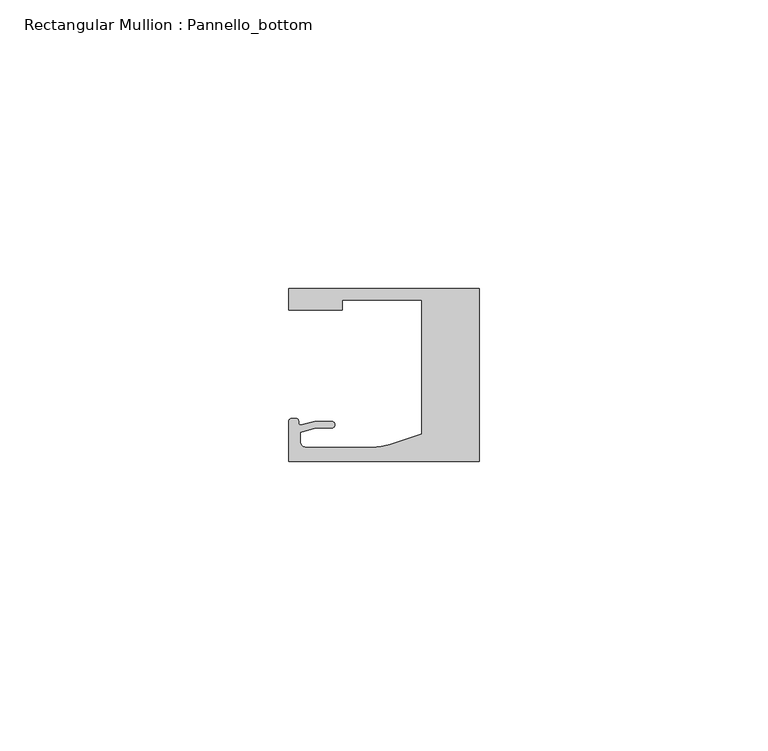
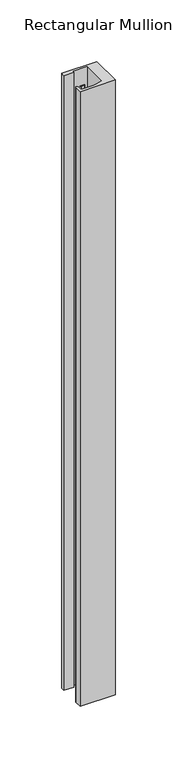
"""IFC4 building model written with IfcOpenShell, lengths in millimetres: member geometry, Rectangular Mullion : Pannello_bottom."""

import ifcopenshell
import ifcopenshell.guid

model = None  # the IFC model being written
_history = None  # IfcOwnerHistory: only IFC2X3 demands one
_inside = {}  # id of a spatial element -> (the spatial element, [elements in it])
_under = {}  # id of a project, library or spatial element -> (it, [spatial elements below it])
_declared = {}  # id of a project -> (the project, [libraries it declares])
_typed = {}  # id of a type object -> (the type object, [elements of that type])
_made_of = {}  # id of a material, layer set ... -> (it, [elements and type objects made of it])


def new_model(schema):
    """Start an empty IFC model of exactly this schema.

    Asked for "IFC4X3", IfcOpenShell would pick the latest addendum, in which some entities
    have other attributes; the version numbers below select the first issue.
    IFC2X3 requires an IfcOwnerHistory on every rooted entity: one is made here for all.
    """
    global model, _history
    if schema == "IFC4X3":
        model = ifcopenshell.file(schema_version=(4, 3, 0, 0))
    else:
        model = ifcopenshell.file(schema=schema)
    _inside.clear()
    _under.clear()
    _declared.clear()
    _typed.clear()
    _made_of.clear()
    _history = None
    if model.schema == "IFC2X3":
        org = make("IfcOrganization", Name="unknown")
        user = make(
            "IfcPersonAndOrganization",
            ThePerson=make("IfcPerson", FamilyName="unknown"),
            TheOrganization=org,
        )
        app = make(
            "IfcApplication",
            ApplicationDeveloper=org,
            Version="unknown",
            ApplicationFullName="unknown",
            ApplicationIdentifier="unknown",
        )
        _history = make(
            "IfcOwnerHistory",
            OwningUser=user,
            OwningApplication=app,
            ChangeAction="ADDED",
            CreationDate=0,
        )
    return model


def make(cls, **values):
    """One entity of the class cls with the attributes given. An attribute that is None is left unset."""
    return model.create_entity(
        cls, **{name: value for name, value in values.items() if value is not None}
    )


def rooted(cls, **values):
    """An entity with a GlobalId (a new one), such as an element, a storey or a relation."""
    return make(cls, GlobalId=ifcopenshell.guid.new(), OwnerHistory=_history, **values)


def si_unit(unit_type, name, prefix=None):
    """IfcSIUnit, for example si_unit("LENGTHUNIT", "METRE", prefix="MILLI")."""
    return make("IfcSIUnit", UnitType=unit_type, Prefix=prefix, Name=name)


def assignment(units):
    """IfcUnitAssignment: the units of a project."""
    return None if units is None else make("IfcUnitAssignment", Units=units)


def point(xyz):
    """IfcCartesianPoint."""
    return None if xyz is None else make("IfcCartesianPoint", Coordinates=xyz)


def direction(xyz):
    """IfcDirection."""
    return None if xyz is None else make("IfcDirection", DirectionRatios=xyz)


def frame(location, z_axis=None, x_axis=None):
    """IfcAxis2Placement3D, a coordinate frame: its origin and axes. An axis left out is left unset."""
    return make(
        "IfcAxis2Placement3D",
        Location=point(location),
        Axis=direction(z_axis),
        RefDirection=direction(x_axis),
    )


def origin():
    """The frame at (0, 0, 0) with its axes left unset."""
    return frame((0.0, 0.0, 0.0))


def place(relative_to, where):
    """IfcLocalPlacement: puts the frame where relative to a parent placement (None: the world)."""
    return make(
        "IfcLocalPlacement", PlacementRelTo=relative_to, RelativePlacement=where
    )


def context(
    kind, dimensions, precision=None, world=None, true_north=None, identifier=None
):
    """IfcGeometricRepresentationContext, for example the 3D "Model" context."""
    return make(
        "IfcGeometricRepresentationContext",
        ContextIdentifier=identifier,
        ContextType=kind,
        CoordinateSpaceDimension=dimensions,
        Precision=precision,
        WorldCoordinateSystem=world,
        TrueNorth=true_north,
    )


def project(units=None, contexts=None):
    """IfcProject with its units and contexts."""
    return rooted(
        "IfcProject",
        Name="project",
        RepresentationContexts=contexts,
        UnitsInContext=assignment(units),
    )


def spatial(cls, under=None, at=None, **own):
    """A site, building, storey or space (cls), placed at a placement, below another one or the project."""
    s = rooted(cls, ObjectPlacement=at, **own)
    if under is not None:
        _under.setdefault(under.id(), (under, []))[1].append(s)
    return s


def polyline(points):
    """IfcPolyline through the points."""
    return make("IfcPolyline", Points=[point(p) for p in points])


def circle_curve(where, radius):
    """IfcCircle in the frame where."""
    return make("IfcCircle", Position=where, Radius=radius)


def shape(context_of_items, identifier, shape_type, items):
    """IfcShapeRepresentation: the items that make up one representation, for example the "Body"."""
    return make(
        "IfcShapeRepresentation",
        ContextOfItems=context_of_items,
        RepresentationIdentifier=identifier,
        RepresentationType=shape_type,
        Items=items,
    )


def source(mapping_origin, context_of_items, identifier, shape_type, items):
    """IfcRepresentationMap: a shape defined once, which mapped items show again and again."""
    return make(
        "IfcRepresentationMap",
        MappingOrigin=mapping_origin,
        MappedRepresentation=shape(context_of_items, identifier, shape_type, items),
    )


def transform(
    local_origin,
    x_axis=None,
    y_axis=None,
    z_axis=None,
    scale=None,
    scale2=None,
    scale3=None,
    uniform=True,
):
    """IfcCartesianTransformationOperator3D, or its non-uniform kind. x_axis, y_axis, z_axis: its Axis1, 2, 3."""
    if uniform:
        return make(
            "IfcCartesianTransformationOperator3D",
            Axis1=direction(x_axis),
            Axis2=direction(y_axis),
            LocalOrigin=point(local_origin),
            Scale=scale,
            Axis3=direction(z_axis),
        )
    return make(
        "IfcCartesianTransformationOperator3DnonUniform",
        Axis1=direction(x_axis),
        Axis2=direction(y_axis),
        LocalOrigin=point(local_origin),
        Scale=scale,
        Axis3=direction(z_axis),
        Scale2=scale2,
        Scale3=scale3,
    )


def mapped(mapping_source, mapping_target):
    """IfcMappedItem: shows the shape of a source again, moved by a transform."""
    return make(
        "IfcMappedItem", MappingSource=mapping_source, MappingTarget=mapping_target
    )


def made_of(thing, what):
    """Note that an element or type object is made of a material, layer set ...; save() writes the relation."""
    if what is not None:
        _made_of.setdefault(what.id(), (what, []))[1].append(thing)
    return thing


def element(
    cls,
    number,
    at=None,
    inside=None,
    cuts=None,
    type_object=None,
    material=None,
    context=None,
    identifier="Body",
    shape_type=None,
    held_by="IfcProductDefinitionShape",
    body=None,
    shapes=None,
    **own,
):
    """One element of the class cls, such as IfcWall. Its Tag is "e" and its number.

    at: its placement. inside: the storey or other place that contains it. cuts: it is an
    opening in that element (IfcRelVoidsElement). A single representation is given by context,
    identifier, shape_type and body (its items); several are given by shapes. held_by: the class
    of the entity that holds the representations. save() writes the other relations.
    """
    e = rooted(cls, Tag="e%d" % number, ObjectPlacement=at, **own)
    if body is not None:
        shapes = [shape(context, identifier, shape_type, body)]
    if shapes is not None:
        e.Representation = make(held_by, Representations=shapes)
    if inside is not None:
        _inside.setdefault(inside.id(), (inside, []))[1].append(e)
    if cuts is not None:
        rooted(
            "IfcRelVoidsElement", RelatingBuildingElement=cuts, RelatedOpeningElement=e
        )
    if type_object is not None:
        _typed.setdefault(type_object.id(), (type_object, []))[1].append(e)
    return made_of(e, material)


def aggregate(whole, parts):
    """IfcRelAggregates: a whole, such as a stair, and the parts it consists of."""
    return rooted("IfcRelAggregates", RelatingObject=whole, RelatedObjects=parts)


def save(model, path):
    """Write the relations noted so far, then the file.

    IfcRelAggregates (storeys below a building ...), IfcRelContainedInSpatialStructure (elements
    in a storey), IfcRelDefinesByType, IfcRelAssociatesMaterial and IfcRelDeclares: one each for
    every whole, place, type object, material and project.
    """
    for whole, parts in _under.values():
        aggregate(whole, parts)
    for where, things in _inside.values():
        rooted(
            "IfcRelContainedInSpatialStructure",
            RelatedElements=things,
            RelatingStructure=where,
        )
    for kind, things in _typed.values():
        rooted("IfcRelDefinesByType", RelatedObjects=things, RelatingType=kind)
    for what, things in _made_of.values():
        rooted("IfcRelAssociatesMaterial", RelatedObjects=things, RelatingMaterial=what)
    for by, libraries in _declared.values():
        rooted("IfcRelDeclares", RelatingContext=by, RelatedDefinitions=libraries)
    model.write(path)


def plane_surface(at):
    """IfcPlane: the flat surface through the origin of the frame at, square to its z axis."""
    return make("IfcPlane", Position=at)


def cylinder_surface(at, radius):
    """IfcCylindricalSurface: all points at the distance radius from the z axis of the frame at."""
    return make("IfcCylindricalSurface", Position=at, Radius=radius)


def revolved_surface(curve, axis_point, axis_direction):
    """IfcSurfaceOfRevolution: the curve turned about the line through axis_point along axis_direction."""
    return make(
        "IfcSurfaceOfRevolution",
        SweptCurve=make("IfcArbitraryOpenProfileDef", ProfileType="CURVE", Curve=curve),
        AxisPosition=make("IfcAxis1Placement", Location=point(axis_point), Axis=direction(axis_direction)),
    )


def extruded_surface(curve, direction_of_extrusion, depth):
    """IfcSurfaceOfLinearExtrusion: the curve pushed along a direction by depth."""
    return make(
        "IfcSurfaceOfLinearExtrusion",
        SweptCurve=make("IfcArbitraryOpenProfileDef", ProfileType="CURVE", Curve=curve),
        ExtrudedDirection=direction(direction_of_extrusion),
        Depth=depth,
    )


def spline_curve(degree, points, multiplicities, knots, weights=None):
    """IfcBSplineCurveWithKnots; with weights, IfcRationalBSplineCurveWithKnots."""
    own = dict(
        Degree=degree,
        ControlPointsList=[point(p) for p in points],
        CurveForm="UNSPECIFIED",
        ClosedCurve=False,
        SelfIntersect=False,
        KnotMultiplicities=multiplicities,
        Knots=knots,
        KnotSpec="UNSPECIFIED",
    )
    if weights is None:
        return make("IfcBSplineCurveWithKnots", **own)
    return make("IfcRationalBSplineCurveWithKnots", WeightsData=weights, **own)


def advanced_brep(points, edges, surfaces, faces):
    """IfcAdvancedBrep: a solid bounded by faces that lie on surfaces and meet in shared edges.

    An edge is (start, end): straight between two places in points (the first is 0);
    or (start, end, curve); or (start, end, curve, False) where it runs against its curve.
    A face is (place in surfaces, loops), or (place, loops, False) where it looks against
    its surface's normal. A loop lists edges by number (the first is 1), with a minus sign
    where the edge is run from its end to its start. The first loop is the outer one.
    """
    corners = [point(p) for p in points]
    vertices = [make("IfcVertexPoint", VertexGeometry=c) for c in corners]
    made = []
    for start, end, *more in edges:
        made.append(
            make(
                "IfcEdgeCurve",
                EdgeStart=vertices[start],
                EdgeEnd=vertices[end],
                EdgeGeometry=more[0] if more else make("IfcPolyline", Points=[corners[start], corners[end]]),
                SameSense=more[1] if len(more) > 1 else True,
            )
        )
    hull = []
    for where, loops, *sense in faces:
        bounds = []
        for j, loop in enumerate(loops):
            ring = [make("IfcOrientedEdge", EdgeElement=made[abs(k) - 1], Orientation=k > 0) for k in loop]
            bounds.append(
                make(
                    "IfcFaceOuterBound" if j == 0 else "IfcFaceBound",
                    Bound=make("IfcEdgeLoop", EdgeList=ring),
                    Orientation=True,
                )
            )
        hull.append(make("IfcAdvancedFace", Bounds=bounds, FaceSurface=surfaces[where], SameSense=sense[0] if sense else True))
    return make("IfcAdvancedBrep", Outer=make("IfcClosedShell", CfsFaces=hull))


def rectangular_mullion_pannello_bottom_8fd7da32(model_context):
    return source(origin(), model_context, "Body", "AdvancedBrep", [
        advanced_brep(
        [(-33.0, 15.0, 0.0), (-33.0, 11.3000004, 0.0), (-23.700041, 11.3000004, 0.0), (-23.700041, 13.0000004, 0.0), (-9.9999723, 13.0000004, 0.0), (-9.9999723, -10.2367227, 0.0), (-15.4591336, -12.0105099, 0.0), (-18.5493024, -12.4999438, 0.0), (-30.0000002, -12.4999419, 0.0), (-31.0, -11.4999419, 0.0), (-31.0, -9.9121746, 0.0), (-28.3419477, -9.1999523, 0.0), (-25.59998, -9.1999523, 0.0), (-25.59998, -7.9999523, 0.0), (-28.4999305, -7.9999523, 0.0), (-30.9223017, -8.6490241, 0.0), (-33.0000135, -8.0000472, 0.0), (-33.0000135, -15.0, 0.0), (0.0, -15.0, 0.0), (0.0, 15.0, 0.0), (-33.0, 15.0, -609.0245992), (0.0, 15.0, -609.0245992), (0.0, -15.0, -609.0245992), (-33.0000135, -15.0, -609.0245992), (-33.0000135, -8.0000472, -609.0245992), (-30.9223017, -8.6490241, -609.0245992), (-28.4999305, -7.9999523, -609.0245992), (-25.59998, -7.9999523, -609.0245992), (-25.59998, -9.1999523, -609.0245992), (-28.3419477, -9.1999523, -609.0245992), (-31.0, -9.9121746, -609.0245992), (-31.0, -11.4999419, -609.0245992), (-30.0000002, -12.4999419, -609.0245992), (-18.5493024, -12.4999438, -609.0245992), (-15.4591336, -12.0105099, -609.0245992), (-9.9999723, -10.2367227, -609.0245992), (-9.9999723, 13.0000004, -609.0245992), (-23.700041, 13.0000004, -609.0245992), (-23.700041, 11.3000004, -609.0245992), (-33.0, 11.3000004, -609.0245992)],
        [
            (0, 1),
            (1, 2),
            (2, 3),
            (3, 4),
            (4, 5),
            (5, 6),
            (6, 7, circle_curve(frame((-18.5493007, -2.4999438, 0.0), z_axis=(0.0, 0.0, -1.0), x_axis=(0.0, -1.0, 0.0)), 10.0)),
            (7, 8),
            (8, 9, circle_curve(frame((-30.0, -11.4999419, 0.0), z_axis=(0.0, 0.0, -1.0), x_axis=(0.0, -1.0, 0.0)), 1.0)),
            (9, 10),
            (10, 11),
            (11, 12),
            (12, 13, circle_curve(frame((-25.59998, -8.5999523, 0.0), z_axis=(0.0, 0.0, 1.0), x_axis=(0.0, -1.0, 0.0)), 0.6)),
            (13, 14),
            (14, 15),
            (15, 16, spline_curve(3, [(-30.9223017, -8.6490241, 0.0), (-31.312054066, -8.717747958, 0.0), (-31.298563602, -8.366228555, 0.0), (-31.305645054, -7.690065204, 0.0), (-31.357433266, -7.563996614, 0.0), (-32.262327879, -7.456527435, 0.0), (-33.0000135, -7.457047519, 0.0), (-33.0000135, -8.0000472, 0.0)], [4, 2, 2, 4], [0.0, 0.001840817752199412, 0.004996616814974408, 0.007702013405570312])),
            (16, 17),
            (17, 18),
            (18, 19),
            (19, 0),
            (20, 21),
            (21, 22),
            (22, 23),
            (23, 24),
            (24, 25, spline_curve(3, [(-33.0000135, -8.0000472, -609.0245992), (-33.0000135, -7.457047519, -609.0245992), (-32.262327879, -7.456527435, -609.0245992), (-31.357433266, -7.563996614, -609.0245992), (-31.305645054, -7.690065204, -609.0245992), (-31.298563602, -8.366228555, -609.0245992), (-31.312054066, -8.717747958, -609.0245992), (-30.9223017, -8.6490241, -609.0245992)], [4, 2, 2, 4], [0.0, 0.0027053965905959043, 0.0058611956533709, 0.007702013405570312])),
            (25, 26),
            (26, 27),
            (27, 28, circle_curve(frame((-25.59998, -8.5999523, -609.0245992), z_axis=(0.0, 0.0, -1.0), x_axis=(0.0, -1.0, 0.0)), 0.6)),
            (28, 29),
            (29, 30),
            (30, 31),
            (31, 32, circle_curve(frame((-30.0, -11.4999419, -609.0245992), z_axis=(0.0, 0.0, 1.0), x_axis=(0.0, -1.0, 0.0)), 1.0)),
            (32, 33),
            (33, 34, circle_curve(frame((-18.5493007, -2.4999438, -609.0245992), z_axis=(0.0, 0.0, 1.0), x_axis=(0.0, -1.0, 0.0)), 10.0)),
            (34, 35),
            (35, 36),
            (36, 37),
            (37, 38),
            (38, 39),
            (39, 20),
            (0, 20),
            (39, 1),
            (38, 2),
            (37, 3),
            (36, 4),
            (35, 5),
            (34, 6),
            (33, 7),
            (32, 8),
            (31, 9),
            (30, 10),
            (29, 11),
            (28, 12),
            (27, 13),
            (26, 14),
            (25, 15),
            (24, 16),
            (23, 17),
            (22, 18),
            (21, 19),
        ],
        [
            plane_surface(frame((0.0, -36.2491502, 0.0), z_axis=(0.0, 0.0, 1.0), x_axis=(-1.0, 0.0, 0.0))),
            plane_surface(frame((0.0, -36.2491502, -609.0245992), z_axis=(0.0, 0.0, -1.0), x_axis=(-1.0, 0.0, 0.0))),
            plane_surface(frame((-33.0, 15.0, 0.0), z_axis=(-1.0, 0.0, 0.0), x_axis=(0.0, 0.0, -1.0))),
            plane_surface(frame((-33.0, 11.3000004, 0.0), z_axis=(0.0, -1.0, 0.0), x_axis=(0.0, 0.0, -1.0))),
            plane_surface(frame((-23.700041, 11.3000004, 0.0), z_axis=(1.0, 0.0, 0.0), x_axis=(0.0, 0.0, -1.0))),
            plane_surface(frame((-23.700041, 13.0000004, 0.0), z_axis=(0.0, -1.0, 0.0), x_axis=(0.0, 0.0, -1.0))),
            plane_surface(frame((-9.9999723, 13.0000004, 0.0), z_axis=(-1.0, 0.0, 0.0), x_axis=(0.0, 0.0, -1.0))),
            plane_surface(frame((-9.9999723, -10.2367227, 0.0), z_axis=(-0.30901670911956314, 0.9510566089801992, 0.0), x_axis=(0.0, 0.0, -1.0))),
            revolved_surface(polyline([(-18.5493007, -12.4999438, -609.0245992), (-18.5493007, -12.4999438, 0.0)]), (-18.5493007, -2.4999438, 0.0), (0.0, 0.0, -1.0)),
            plane_surface(frame((-18.5493024, -12.4999438, 0.0), z_axis=(1.6923026533778639e-07, 0.9999999999999858, 0.0), x_axis=(0.0, 0.0, -1.0))),
            revolved_surface(polyline([(-30.0, -12.4999419, -609.0245992), (-30.0, -12.4999419, 0.0)]), (-30.0, -11.4999419, 0.0), (0.0, 0.0, -1.0)),
            plane_surface(frame((-31.0, -11.4999419, 0.0), z_axis=(1.0, 0.0, 0.0), x_axis=(0.0, 0.0, -1.0))),
            plane_surface(frame((-31.0, -9.9121746, 0.0), z_axis=(0.25881883204288636, -0.9659258833782002, 0.0), x_axis=(0.0, 0.0, -1.0))),
            plane_surface(frame((-28.3419477, -9.1999523, 0.0), z_axis=(0.0, -1.0, 0.0), x_axis=(0.0, 0.0, -1.0))),
            cylinder_surface(frame((-25.59998, -8.5999523, 0.0), z_axis=(0.0, 0.0, 1.0), x_axis=(0.0, -1.0, 0.0)), 0.6),
            plane_surface(frame((-25.59998, -7.9999523, 0.0), z_axis=(0.0, 1.0, 0.0), x_axis=(0.0, 0.0, -1.0))),
            plane_surface(frame((-28.4999305, -7.9999523, 0.0), z_axis=(-0.25881883200192934, 0.9659258833891746, 0.0), x_axis=(0.0, 0.0, -1.0))),
            extruded_surface(spline_curve(3, [(-30.9223017, -8.6490241, -609.0245992), (-31.312054066, -8.717747958, -609.0245992), (-31.298563602, -8.366228555, -609.0245992), (-31.305645054, -7.690065204, -609.0245992), (-31.357433266, -7.563996614, -609.0245992), (-32.262327879, -7.456527435, -609.0245992), (-33.0000135, -7.457047519, -609.0245992), (-33.0000135, -8.0000472, -609.0245992)], [4, 2, 2, 4], [0.0, 0.001840817752199412, 0.004996616814974408, 0.007702013405570312]), (0.0, 0.0, 609.0245992), 609.0245992),
            plane_surface(frame((-33.0000135, -8.0000472, 0.0), z_axis=(-1.0, 0.0, 0.0), x_axis=(0.0, 0.0, -1.0))),
            plane_surface(frame((-33.0000135, -15.0, 0.0), z_axis=(0.0, -1.0, 0.0), x_axis=(0.0, 0.0, -1.0))),
            plane_surface(frame((0.0, -15.0, 0.0), z_axis=(1.0, 0.0, 0.0), x_axis=(0.0, 0.0, -1.0))),
            plane_surface(frame((0.0, 15.0, 0.0), z_axis=(0.0, 1.0, 0.0), x_axis=(0.0, 0.0, -1.0))),
        ],
        [
            (0, [[1, 2, 3, 4, 5, 6, 7, 8, 9, 10, 11, 12, 13, 14, 15, 16, 17, 18, 19, 20]]),
            (1, [[21, 22, 23, 24, 25, 26, 27, 28, 29, 30, 31, 32, 33, 34, 35, 36, 37, 38, 39, 40]]),
            (2, [[-1, 41, -40, 42]]),
            (3, [[-2, -42, -39, 43]]),
            (4, [[-3, -43, -38, 44]]),
            (5, [[-4, -44, -37, 45]]),
            (6, [[-5, -45, -36, 46]]),
            (7, [[-6, -46, -35, 47]]),
            (8, [[-7, -47, -34, 48]]),
            (9, [[-8, -48, -33, 49]]),
            (10, [[-9, -49, -32, 50]]),
            (11, [[-10, -50, -31, 51]]),
            (12, [[-11, -51, -30, 52]]),
            (13, [[-12, -52, -29, 53]]),
            (14, [[-13, -53, -28, 54]]),
            (15, [[-14, -54, -27, 55]]),
            (16, [[-15, -55, -26, 56]]),
            (17, [[-16, -56, -25, 57]]),
            (18, [[-17, -57, -24, 58]]),
            (19, [[-18, -58, -23, 59]]),
            (20, [[-19, -59, -22, 60]]),
            (21, [[-20, -60, -21, -41]]),
        ],
    ),
    ])


if __name__ == "__main__":
    model = new_model("IFC4")
    model_context = context("Model", 3, world=origin())
    ifc_project = project(units=[si_unit("LENGTHUNIT", "METRE", prefix="MILLI")], contexts=[model_context])
    site = spatial("IfcSite", under=ifc_project)
    building = spatial("IfcBuilding", under=site)
    placement = place(None, origin())
    rectangular_mullion_pannello_bottom_shape = rectangular_mullion_pannello_bottom_8fd7da32(model_context)
    element("IfcMember", 1, ObjectType="Rectangular Mullion : Pannello_bottom", at=placement, inside=building, context=model_context, shape_type="MappedRepresentation", body=[
        mapped(rectangular_mullion_pannello_bottom_shape, transform((0.0, 0.0, 0.0), x_axis=(1.0, 0.0, 0.0), y_axis=(0.0, 1.0, 0.0), z_axis=(0.0, 0.0, 1.0))),
    ])
    save(model, "model.ifc")

# Revit data of these elements
# Type "Rectangular Mullion : Pannello_bottom"
#   built-in parameter 1007322 = 0.0984252 (stored number, unit not read)
#   built-in parameter 1007321 = 0.0328083 (stored number, unit not read)
#   built-in parameter 1007320 = 0 (stored number, unit not read)
